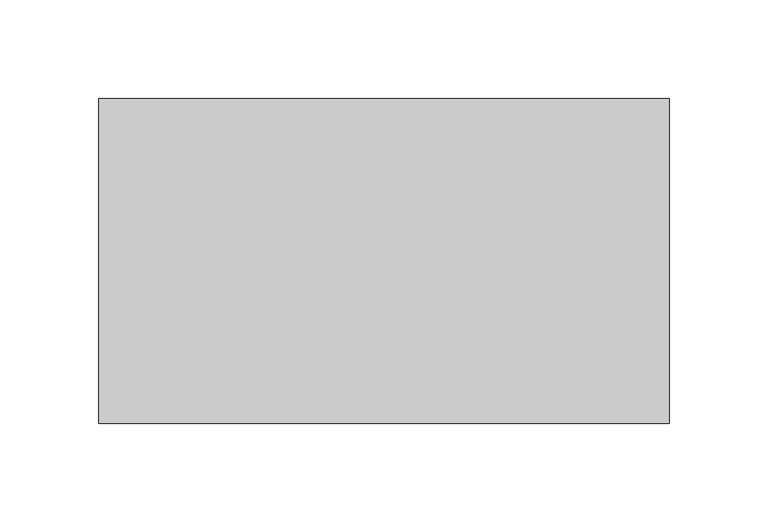
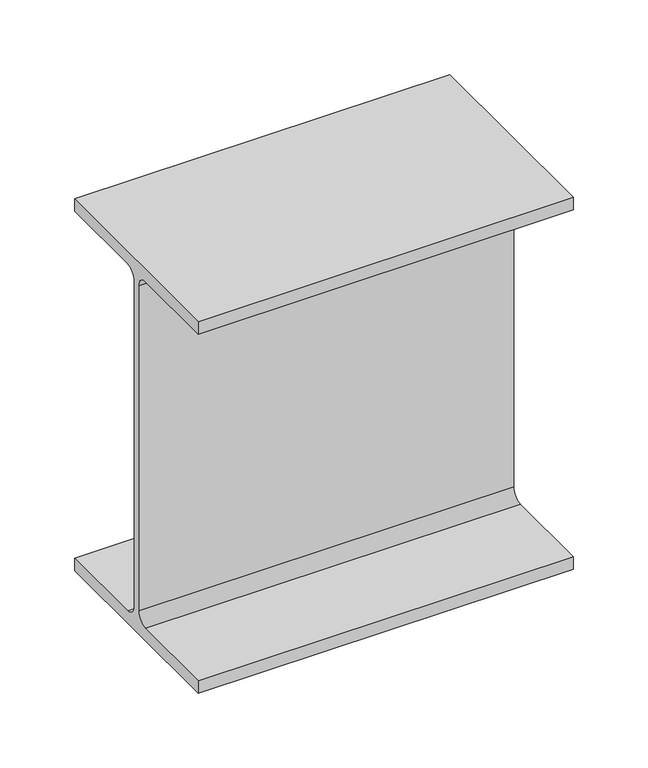
"""IFC4 building model written with IfcOpenShell, lengths in millimetres: beam geometry, Old_Steel Beam_H-KSD3502 : H_SB_ASB_H-300×150x6.5x9."""

from ifc_helpers import new_model, si_unit, point, frame, frame_2d, origin, place, context, project, spatial, polyline, circle_curve, trimmed, segment, composite_curve, outline, extrude, source, transform, mapped, element, save


def beam_91cecbf6(model_context):
    return source(origin(), model_context, "Body", "SweptSolid", [
        extrude(outline(composite_curve([segment(polyline([(82.5, -141.5), (82.5, -151.7), (-82.5, -151.7), (-82.5, -141.5), (-11.9, -141.5)]), True, "CONTINUOUS"), segment(trimmed(circle_curve(frame_2d((-11.9, -132.6)), 8.9), [point((-11.9, -141.5))], [point((-3.0, -132.6))], True, "CARTESIAN"), True, "CONTINUOUS"), segment(polyline([(-3.0, -132.6), (-3.0, 132.6)]), True, "CONTINUOUS"), segment(trimmed(circle_curve(frame_2d((-11.9, 132.6)), 8.9), [point((-3.0, 132.6))], [point((-11.9, 141.5))], True, "CARTESIAN"), True, "CONTINUOUS"), segment(polyline([(-11.9, 141.5), (-82.5, 141.5), (-82.5, 151.7), (82.5, 151.7), (82.5, 141.5), (11.9, 141.5)]), True, "CONTINUOUS"), segment(trimmed(circle_curve(frame_2d((11.9, 132.6)), 8.9), [point((11.9, 141.5))], [point((3.0, 132.6))], True, "CARTESIAN"), True, "CONTINUOUS"), segment(polyline([(3.0, 132.6), (3.0, -132.6)]), True, "CONTINUOUS"), segment(trimmed(circle_curve(frame_2d((11.9, -132.6)), 8.9), [point((3.0, -132.6))], [point((11.9, -141.5))], True, "CARTESIAN"), True, "CONTINUOUS"), segment(polyline([(11.9, -141.5), (82.5, -141.5)]), True, "CONTINUOUS")], self_intersect=False)), frame((-7.3, 0.0, 0.0), z_axis=(1.0, 0.0, 0.0), x_axis=(0.0, 1.0, 0.0)), (0.0, 0.0, 1.0), 289.6),
    ])


if __name__ == "__main__":
    model = new_model("IFC4")
    model_context = context("Model", 3, world=origin())
    ifc_project = project(units=[si_unit("LENGTHUNIT", "METRE", prefix="MILLI")], contexts=[model_context])
    site = spatial("IfcSite", under=ifc_project)
    building = spatial("IfcBuilding", under=site)
    placement = place(None, origin())
    beam_shape = beam_91cecbf6(model_context)
    element("IfcBeam", 1, ObjectType="Old_Steel Beam_H-KSD3502 : H_SB_ASB_H-300×150x6.5x9", at=placement, inside=building, context=model_context, shape_type="MappedRepresentation", body=[
        mapped(beam_shape, transform((0.0, 0.0, 0.0), x_axis=(1.0, 0.0, 0.0), y_axis=(0.0, 1.0, 0.0), z_axis=(0.0, 0.0, 1.0))),
    ])
    save(model, "model.ifc")

# Revit data of these elements
# Type "Old_Steel Beam_H-KSD3502 : H_SB_ASB_H-300×150x6.5x9"
#   Width = 15.0 cm
#   Web Thickness = 0.65 cm
#   Web Fillet = 1.3 cm
#   Warping Constant = 107174.0 cm⁶
#   Torsional Moment of Inertia = 9.9539 cm⁴
#   Torsional Modulus = 1.0 cm³
#   Section Area = 46.78 cm²
#   Plastic Modulus weak axis = 105.0 cm³
#   Plastic Modulus strong axis = 542.0 cm³
#   Perimeter = 1.17 m²/m
#   Nominal Weight = 36.70 kgf/m
#   Moment of Inertia weak axis = 508.00 cm⁴
#   Moment of Inertia strong axis = 7210.00 cm⁴
#   Height = 30.0 cm
#   Flange Thickness = 0.9 cm
#   Elastic Modulus weak axis = 67.7 cm³
#   Elastic Modulus strong axis = 481.0 cm³
#   Centroid Vertical = 15.0 cm
#   Centroid Horizontal = 7.5 cm
#   Length [instance default] = 1.5240 m
#   Structural Material [instance default] = Steel, 45-345
#   Assembly Code = ""
# Element 1 (IfcBeam, "Old_Steel Beam_H-KSD3502 : H_SB_ASB_H-300×150x6.5x9")
#   Structural Material = none
# Materials
#   "Steel, 45-345": class "Metal", colour RGB 189 187 185, transparency 0, Description = "Steel 345 MPa", Cost = 0
